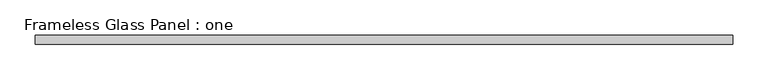
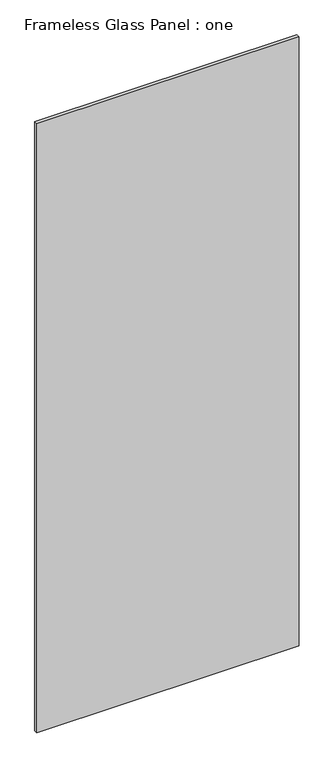
"""IFC4 building model written with IfcOpenShell, lengths in millimetres: plate geometry, Frameless Glass Panel : one."""

from ifc_helpers import new_model, si_unit, origin, origin_with_axes, place, context, project, spatial, polyline, outline, extrude, source, transform, mapped, element, save


def frameless_glass_panel_one_686ffde2(model_context):
    return source(origin(), model_context, "Body", "SweptSolid", [
        extrude(outline(polyline([(496.3583333, -6.35), (-496.3583333, -6.35), (-496.3583333, 6.35), (496.3583333, 6.35), (496.3583333, -6.35)])), origin_with_axes(), (0.0, 0.0, 1.0), 2438.4),
    ])


if __name__ == "__main__":
    model = new_model("IFC4")
    model_context = context("Model", 3, world=origin())
    ifc_project = project(units=[si_unit("LENGTHUNIT", "METRE", prefix="MILLI")], contexts=[model_context])
    site = spatial("IfcSite", under=ifc_project)
    building = spatial("IfcBuilding", under=site)
    placement = place(None, origin())
    frameless_glass_panel_one_shape = frameless_glass_panel_one_686ffde2(model_context)
    element("IfcPlate", 1, ObjectType="Frameless Glass Panel : one", at=placement, inside=building, context=model_context, shape_type="MappedRepresentation", body=[
        mapped(frameless_glass_panel_one_shape, transform((0.0, 0.0, 0.0), x_axis=(1.0, 0.0, 0.0), y_axis=(0.0, 1.0, 0.0), z_axis=(0.0, 0.0, 1.0))),
    ])
    save(model, "model.ifc")

# Revit data of these elements
# Type "Frameless Glass Panel : one"
#   Glass Thickness = 0' - 0 1/2"
#   Gap btwn Panels = 0' - 0 1/4"
#   Panel Material = TEMPERED GLASS DOOR/SIDELIGHT TO MATCH EXISTING CONF. ROOM
# Element 1 (IfcPlate, "Frameless Glass Panel : one")
#   Materials on its faces: "TEMPERED GLASS DOOR/SIDELIGHT TO MATCH EXISTING CONF. ROOM"
# Materials
#   "TEMPERED GLASS DOOR/SIDELIGHT TO MATCH EXISTING CONF. ROOM": class "Glass", colour RGB 218 227 224, transparency 0.85, Description = "Soda Lime Glass", Cost = 0
